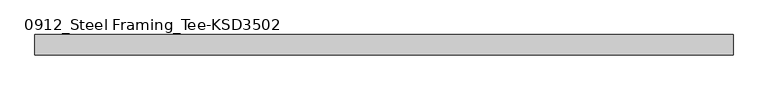
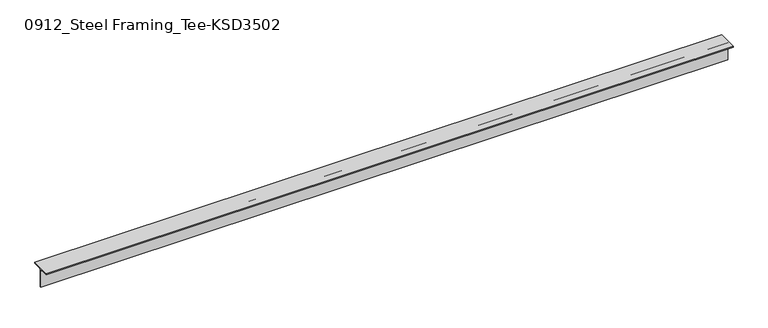
"""IFC4 building model written with IfcOpenShell, lengths in millimetres: member geometry, 0912_Steel Framing_Tee-KSD3502 : H_SB_ASB_CT-150x150x6.5x9."""

import ifcopenshell
import ifcopenshell.guid

model = None  # the IFC model being written
_history = None  # IfcOwnerHistory: only IFC2X3 demands one
_inside = {}  # id of a spatial element -> (the spatial element, [elements in it])
_under = {}  # id of a project, library or spatial element -> (it, [spatial elements below it])
_declared = {}  # id of a project -> (the project, [libraries it declares])
_typed = {}  # id of a type object -> (the type object, [elements of that type])
_made_of = {}  # id of a material, layer set ... -> (it, [elements and type objects made of it])


def new_model(schema):
    """Start an empty IFC model of exactly this schema.

    Asked for "IFC4X3", IfcOpenShell would pick the latest addendum, in which some entities
    have other attributes; the version numbers below select the first issue.
    IFC2X3 requires an IfcOwnerHistory on every rooted entity: one is made here for all.
    """
    global model, _history
    if schema == "IFC4X3":
        model = ifcopenshell.file(schema_version=(4, 3, 0, 0))
    else:
        model = ifcopenshell.file(schema=schema)
    _inside.clear()
    _under.clear()
    _declared.clear()
    _typed.clear()
    _made_of.clear()
    _history = None
    if model.schema == "IFC2X3":
        org = make("IfcOrganization", Name="unknown")
        user = make(
            "IfcPersonAndOrganization",
            ThePerson=make("IfcPerson", FamilyName="unknown"),
            TheOrganization=org,
        )
        app = make(
            "IfcApplication",
            ApplicationDeveloper=org,
            Version="unknown",
            ApplicationFullName="unknown",
            ApplicationIdentifier="unknown",
        )
        _history = make(
            "IfcOwnerHistory",
            OwningUser=user,
            OwningApplication=app,
            ChangeAction="ADDED",
            CreationDate=0,
        )
    return model


def make(cls, **values):
    """One entity of the class cls with the attributes given. An attribute that is None is left unset."""
    return model.create_entity(
        cls, **{name: value for name, value in values.items() if value is not None}
    )


def rooted(cls, **values):
    """An entity with a GlobalId (a new one), such as an element, a storey or a relation."""
    return make(cls, GlobalId=ifcopenshell.guid.new(), OwnerHistory=_history, **values)


def si_unit(unit_type, name, prefix=None):
    """IfcSIUnit, for example si_unit("LENGTHUNIT", "METRE", prefix="MILLI")."""
    return make("IfcSIUnit", UnitType=unit_type, Prefix=prefix, Name=name)


def assignment(units):
    """IfcUnitAssignment: the units of a project."""
    return None if units is None else make("IfcUnitAssignment", Units=units)


def point(xyz):
    """IfcCartesianPoint."""
    return None if xyz is None else make("IfcCartesianPoint", Coordinates=xyz)


def direction(xyz):
    """IfcDirection."""
    return None if xyz is None else make("IfcDirection", DirectionRatios=xyz)


def frame(location, z_axis=None, x_axis=None):
    """IfcAxis2Placement3D, a coordinate frame: its origin and axes. An axis left out is left unset."""
    return make(
        "IfcAxis2Placement3D",
        Location=point(location),
        Axis=direction(z_axis),
        RefDirection=direction(x_axis),
    )


def frame_2d(location, x_axis=None):
    """IfcAxis2Placement2D, a coordinate frame in the plane: its origin and x axis."""
    return make(
        "IfcAxis2Placement2D", Location=point(location), RefDirection=direction(x_axis)
    )


def origin():
    """The frame at (0, 0, 0) with its axes left unset."""
    return frame((0.0, 0.0, 0.0))


def place(relative_to, where):
    """IfcLocalPlacement: puts the frame where relative to a parent placement (None: the world)."""
    return make(
        "IfcLocalPlacement", PlacementRelTo=relative_to, RelativePlacement=where
    )


def context(
    kind, dimensions, precision=None, world=None, true_north=None, identifier=None
):
    """IfcGeometricRepresentationContext, for example the 3D "Model" context."""
    return make(
        "IfcGeometricRepresentationContext",
        ContextIdentifier=identifier,
        ContextType=kind,
        CoordinateSpaceDimension=dimensions,
        Precision=precision,
        WorldCoordinateSystem=world,
        TrueNorth=true_north,
    )


def project(units=None, contexts=None):
    """IfcProject with its units and contexts."""
    return rooted(
        "IfcProject",
        Name="project",
        RepresentationContexts=contexts,
        UnitsInContext=assignment(units),
    )


def spatial(cls, under=None, at=None, **own):
    """A site, building, storey or space (cls), placed at a placement, below another one or the project."""
    s = rooted(cls, ObjectPlacement=at, **own)
    if under is not None:
        _under.setdefault(under.id(), (under, []))[1].append(s)
    return s


def polyline(points):
    """IfcPolyline through the points."""
    return make("IfcPolyline", Points=[point(p) for p in points])


def circle_curve(where, radius):
    """IfcCircle in the frame where."""
    return make("IfcCircle", Position=where, Radius=radius)


def trimmed(basis, trim1, trim2, sense, master):
    """IfcTrimmedCurve: the piece of a basis curve between two trims."""
    return make(
        "IfcTrimmedCurve",
        BasisCurve=basis,
        Trim1=trim1,
        Trim2=trim2,
        SenseAgreement=sense,
        MasterRepresentation=master,
    )


def segment(curve, same_sense, transition):
    """IfcCompositeCurveSegment."""
    return make(
        "IfcCompositeCurveSegment",
        Transition=transition,
        SameSense=same_sense,
        ParentCurve=curve,
    )


def composite_curve(segments, self_intersect=None):
    """IfcCompositeCurve: segments joined end to end."""
    return make("IfcCompositeCurve", Segments=segments, SelfIntersect=self_intersect)


def outline(outer, holes=None, kind="AREA"):
    """IfcArbitraryClosedProfileDef: a profile drawn as a closed curve; with holes, ...WithVoids."""
    if holes is None:
        return make("IfcArbitraryClosedProfileDef", ProfileType=kind, OuterCurve=outer)
    return make(
        "IfcArbitraryProfileDefWithVoids",
        ProfileType=kind,
        OuterCurve=outer,
        InnerCurves=holes,
    )


def extrude(swept, where, along, depth):
    """IfcExtrudedAreaSolid: the profile swept, set in the frame where, extruded along a direction by depth."""
    return make(
        "IfcExtrudedAreaSolid",
        SweptArea=swept,
        Position=where,
        ExtrudedDirection=direction(along),
        Depth=depth,
    )


def shape(context_of_items, identifier, shape_type, items):
    """IfcShapeRepresentation: the items that make up one representation, for example the "Body"."""
    return make(
        "IfcShapeRepresentation",
        ContextOfItems=context_of_items,
        RepresentationIdentifier=identifier,
        RepresentationType=shape_type,
        Items=items,
    )


def source(mapping_origin, context_of_items, identifier, shape_type, items):
    """IfcRepresentationMap: a shape defined once, which mapped items show again and again."""
    return make(
        "IfcRepresentationMap",
        MappingOrigin=mapping_origin,
        MappedRepresentation=shape(context_of_items, identifier, shape_type, items),
    )


def transform(
    local_origin,
    x_axis=None,
    y_axis=None,
    z_axis=None,
    scale=None,
    scale2=None,
    scale3=None,
    uniform=True,
):
    """IfcCartesianTransformationOperator3D, or its non-uniform kind. x_axis, y_axis, z_axis: its Axis1, 2, 3."""
    if uniform:
        return make(
            "IfcCartesianTransformationOperator3D",
            Axis1=direction(x_axis),
            Axis2=direction(y_axis),
            LocalOrigin=point(local_origin),
            Scale=scale,
            Axis3=direction(z_axis),
        )
    return make(
        "IfcCartesianTransformationOperator3DnonUniform",
        Axis1=direction(x_axis),
        Axis2=direction(y_axis),
        LocalOrigin=point(local_origin),
        Scale=scale,
        Axis3=direction(z_axis),
        Scale2=scale2,
        Scale3=scale3,
    )


def mapped(mapping_source, mapping_target):
    """IfcMappedItem: shows the shape of a source again, moved by a transform."""
    return make(
        "IfcMappedItem", MappingSource=mapping_source, MappingTarget=mapping_target
    )


def made_of(thing, what):
    """Note that an element or type object is made of a material, layer set ...; save() writes the relation."""
    if what is not None:
        _made_of.setdefault(what.id(), (what, []))[1].append(thing)
    return thing


def element(
    cls,
    number,
    at=None,
    inside=None,
    cuts=None,
    type_object=None,
    material=None,
    context=None,
    identifier="Body",
    shape_type=None,
    held_by="IfcProductDefinitionShape",
    body=None,
    shapes=None,
    **own,
):
    """One element of the class cls, such as IfcWall. Its Tag is "e" and its number.

    at: its placement. inside: the storey or other place that contains it. cuts: it is an
    opening in that element (IfcRelVoidsElement). A single representation is given by context,
    identifier, shape_type and body (its items); several are given by shapes. held_by: the class
    of the entity that holds the representations. save() writes the other relations.
    """
    e = rooted(cls, Tag="e%d" % number, ObjectPlacement=at, **own)
    if body is not None:
        shapes = [shape(context, identifier, shape_type, body)]
    if shapes is not None:
        e.Representation = make(held_by, Representations=shapes)
    if inside is not None:
        _inside.setdefault(inside.id(), (inside, []))[1].append(e)
    if cuts is not None:
        rooted(
            "IfcRelVoidsElement", RelatingBuildingElement=cuts, RelatedOpeningElement=e
        )
    if type_object is not None:
        _typed.setdefault(type_object.id(), (type_object, []))[1].append(e)
    return made_of(e, material)


def aggregate(whole, parts):
    """IfcRelAggregates: a whole, such as a stair, and the parts it consists of."""
    return rooted("IfcRelAggregates", RelatingObject=whole, RelatedObjects=parts)


def save(model, path):
    """Write the relations noted so far, then the file.

    IfcRelAggregates (storeys below a building ...), IfcRelContainedInSpatialStructure (elements
    in a storey), IfcRelDefinesByType, IfcRelAssociatesMaterial and IfcRelDeclares: one each for
    every whole, place, type object, material and project.
    """
    for whole, parts in _under.values():
        aggregate(whole, parts)
    for where, things in _inside.values():
        rooted(
            "IfcRelContainedInSpatialStructure",
            RelatedElements=things,
            RelatingStructure=where,
        )
    for kind, things in _typed.values():
        rooted("IfcRelDefinesByType", RelatedObjects=things, RelatingType=kind)
    for what, things in _made_of.values():
        rooted("IfcRelAssociatesMaterial", RelatedObjects=things, RelatingMaterial=what)
    for by, libraries in _declared.values():
        rooted("IfcRelDeclares", RelatingContext=by, RelatedDefinitions=libraries)
    model.write(path)


def member_0912_steel_framing_tee_ksd3502_2863cb2a(model_context):
    return source(origin(), model_context, "Body", "SweptSolid", [
        extrude(outline(composite_curve([segment(polyline([(-75.0, 75.0), (75.0, 75.0), (75.0, 66.0), (16.25, 66.0)]), True, "CONTINUOUS"), segment(trimmed(circle_curve(frame_2d((16.25, 53.0)), 13.0), [point((16.25, 66.0))], [point((3.25, 53.0))], True, "CARTESIAN"), True, "CONTINUOUS"), segment(polyline([(3.25, 53.0), (3.25, -75.0), (-3.25, -75.0), (-3.25, 53.0)]), True, "CONTINUOUS"), segment(trimmed(circle_curve(frame_2d((-16.25, 53.0)), 13.0), [point((-3.25, 53.0))], [point((-16.25, 66.0))], True, "CARTESIAN"), True, "CONTINUOUS"), segment(polyline([(-16.25, 66.0), (-75.0, 66.0), (-75.0, 75.0)]), True, "CONTINUOUS")], self_intersect=False)), frame((-2587.75, 0.0, 0.0), z_axis=(1.0, 0.0, 0.0), x_axis=(0.0, 1.0, 0.0)), (0.0, 0.0, 1.0), 5164.8),
    ])


if __name__ == "__main__":
    model = new_model("IFC4")
    model_context = context("Model", 3, world=origin())
    ifc_project = project(units=[si_unit("LENGTHUNIT", "METRE", prefix="MILLI")], contexts=[model_context])
    site = spatial("IfcSite", under=ifc_project)
    building = spatial("IfcBuilding", under=site)
    placement = place(None, origin())
    member_0912_steel_framing_tee_ksd3502_shape = member_0912_steel_framing_tee_ksd3502_2863cb2a(model_context)
    element("IfcMember", 1, ObjectType="0912_Steel Framing_Tee-KSD3502 : H_SB_ASB_CT-150x150x6.5x9", at=placement, inside=building, context=model_context, shape_type="MappedRepresentation", body=[
        mapped(member_0912_steel_framing_tee_ksd3502_shape, transform((0.0, 0.0, 0.0), x_axis=(1.0, 0.0, 0.0), y_axis=(0.0, 1.0, 0.0), z_axis=(0.0, 0.0, 1.0))),
    ])
    save(model, "model.ifc")

# Revit data of these elements
# Type "0912_Steel Framing_Tee-KSD3502 : H_SB_ASB_CT-150x150x6.5x9"
#   H_WM Code_1 = "S01AA003-00001 | Main Steel Structure Fabrication Work | Shelter/Building | Light Steel - Standard (30KG/M>Weight) | Material: (   )"
#   H_WM Code_2 = "S03AA029-00001 | Main Steel Structure Erection Work | Shelter/Building | Light Steel (30KG/M>Weight) | Material: (   )"
#   H_WM Code_3 = "S01AA010-00001 | Main Steel Structure Fabrication Work | Shelter/Building | Steel Painting/Coating | for Non-Fireproofed Steel Surface, Surface Preparation, Primer, Second & Final Coat | Material: (   )"
#   H_Q'ty Cal Type Tag = "SB-Q2"
#   Width = 15.0 cm
#   Web Thickness = 0.65 cm
#   Web Fillet = 1.3 cm
#   Section Area = 23.39 cm²
#   Perimeter = 0.60 m²/m
#   Nominal Weight = 18.40 kgf/m
#   Height = 15.0 cm
#   Flange Thickness = 0.9 cm
#   Centroid Vertical = 7.5 cm
#   Centroid Horizontal = 7.5 cm
#   Length [instance default] = 1.5000 m
#   Structural Material [instance default] = Steel, 45-345
#   Warping Constant = (empty or 0)
#   Torsional Moment of Inertia = 0
#   Section Name Key = ""
#   Plastic Modulus weak axis = 0
#   Plastic Modulus strong axis = 0
#   Moment of Inertia weak axis = 0
#   Moment of Inertia strong axis = 0
#   Elastic Modulus weak axis = 0
#   Elastic Modulus strong axis = 0
#   Bolt Spacing = 0
#   Assembly Code = ""
# Element 1 (IfcMember, "0912_Steel Framing_Tee-KSD3502 : H_SB_ASB_CT-150x150x6.5x9")
#   Structural Material = none
# Materials
#   "Steel, 45-345": class "Metal", colour RGB 189 187 185, transparency 0, Description = "Steel 345 MPa", Cost = 0
